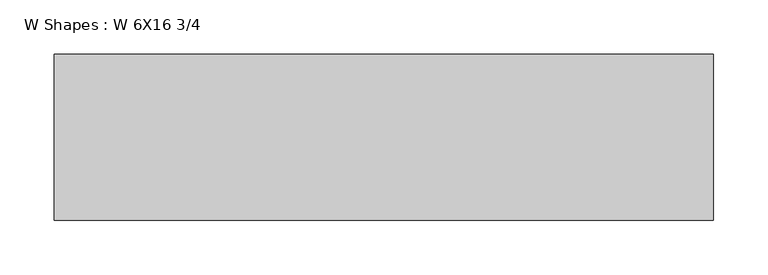
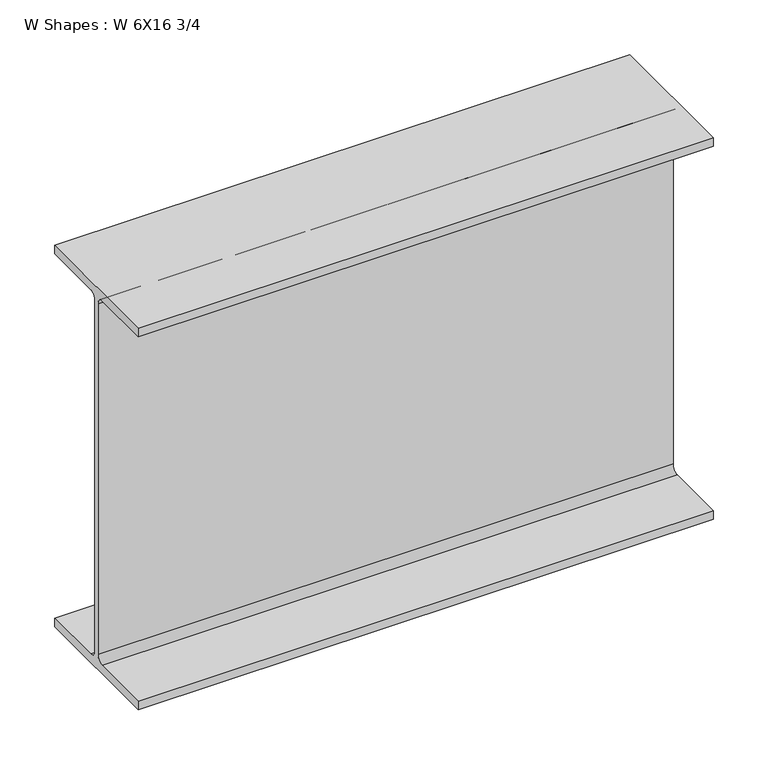
"""IFC4 building model written with IfcOpenShell, lengths in millimetres: beam geometry, W Shapes : W 6X16 3/4."""

from ifc_helpers import new_model, si_unit, point, frame, frame_2d, origin, place, context, project, spatial, polyline, circle_curve, trimmed, segment, composite_curve, outline, extrude, source, transform, mapped, element, save


def w_shapes_w_6x16_3_4_ba0ed1b2(model_context):
    return source(origin(), model_context, "Body", "SweptSolid", [
        extrude(outline(composite_curve([segment(polyline([(76.1964281, -203.073), (76.1964281, -212.725), (-76.2035719, -212.725), (-76.2035719, -203.073), (-10.5445719, -203.073)]), True, "CONTINUOUS"), segment(trimmed(circle_curve(frame_2d((-10.5445719, -195.453)), 7.62), [point((-10.5445719, -203.073))], [point((-2.9245719, -195.453))], True, "CARTESIAN"), True, "CONTINUOUS"), segment(polyline([(-2.9245719, -195.453), (-2.9245719, 195.453)]), True, "CONTINUOUS"), segment(trimmed(circle_curve(frame_2d((-10.5445719, 195.453)), 7.62), [point((-2.9245719, 195.453))], [point((-10.5445719, 203.073))], True, "CARTESIAN"), True, "CONTINUOUS"), segment(polyline([(-10.5445719, 203.073), (-76.2035719, 203.073), (-76.2035719, 212.725), (76.1964281, 212.725), (76.1964281, 203.073), (10.5374281, 203.073)]), True, "CONTINUOUS"), segment(trimmed(circle_curve(frame_2d((10.5374281, 195.453)), 7.62), [point((10.5374281, 203.073))], [point((2.9174281, 195.453))], True, "CARTESIAN"), True, "CONTINUOUS"), segment(polyline([(2.9174281, 195.453), (2.9174281, -195.453)]), True, "CONTINUOUS"), segment(trimmed(circle_curve(frame_2d((10.5374281, -195.453)), 7.62), [point((2.9174281, -195.453))], [point((10.5374281, -203.073))], True, "CARTESIAN"), True, "CONTINUOUS"), segment(polyline([(10.5374281, -203.073), (76.1964281, -203.073)]), True, "CONTINUOUS")], self_intersect=False)), frame((-303.1556375, 0.0, 0.0), z_axis=(1.0, 0.0, 0.0), x_axis=(0.0, 1.0, 0.0)), (0.0, 0.0, 1.0), 606.311275),
    ])


if __name__ == "__main__":
    model = new_model("IFC4")
    model_context = context("Model", 3, world=origin())
    ifc_project = project(units=[si_unit("LENGTHUNIT", "METRE", prefix="MILLI")], contexts=[model_context])
    site = spatial("IfcSite", under=ifc_project)
    building = spatial("IfcBuilding", under=site)
    placement = place(None, origin())
    w_shapes_w_6x16_3_4_shape = w_shapes_w_6x16_3_4_ba0ed1b2(model_context)
    element("IfcBeam", 1, ObjectType="W Shapes : W 6X16 3/4", at=placement, inside=building, context=model_context, shape_type="MappedRepresentation", body=[
        mapped(w_shapes_w_6x16_3_4_shape, transform((0.0, 0.0, 0.0), x_axis=(1.0, 0.0, 0.0), y_axis=(0.0, 1.0, 0.0), z_axis=(0.0, 0.0, 1.0))),
    ])
    save(model, "model.ifc")

# Revit data of these elements
# Type "W Shapes : W 6X16 3/4"
#   Section Name Key = "W12x26"
#   Assembly Code = "B10"
#   Width = 152.4 mm
#   Web Thickness = 5.842 mm
#   Web Fillet = 7.62 mm
#   Warping Constant = 163001.3 cm⁶
#   Torsional Moment of Inertia = 12.4869 cm⁴
#   Section Area = 7.65 in²
#   Plastic Modulus weak axis = 0.00472801 (stored number, unit not read)
#   Plastic Modulus strong axis = 0.0215278 (stored number, unit not read)
#   Perimeter = 15.0571 m²/m
#   Nominal Weight = 379.441 N/m
#   Moment of Inertia weak axis = 720.08 cm⁴
#   Moment of Inertia strong axis = 8491.12 cm⁴
#   Height = 425.45 mm
#   Flange Thickness = 9.652 mm
#   Elastic Modulus weak axis = 0.00309028 (stored number, unit not read)
#   Elastic Modulus strong axis = 0.0193287 (stored number, unit not read)
#   Centroid Vertical = 212.725 mm
#   Centroid Horizontal = 76.2 mm
#   Length [instance default] = 5' - 0"
#   Structural Material [instance default] = Steel ASTM A992
#   Principal Axes Angle = 0
# Element 1 (IfcBeam, "W Shapes : W 6X16 3/4")
#   Materials on its faces: "Steel ASTM A992"
# Materials
#   "Steel ASTM A992": class "Metal", colour RGB 189 187 185, transparency 0, Description = "Structural steel 50ksi", Cost = 0
